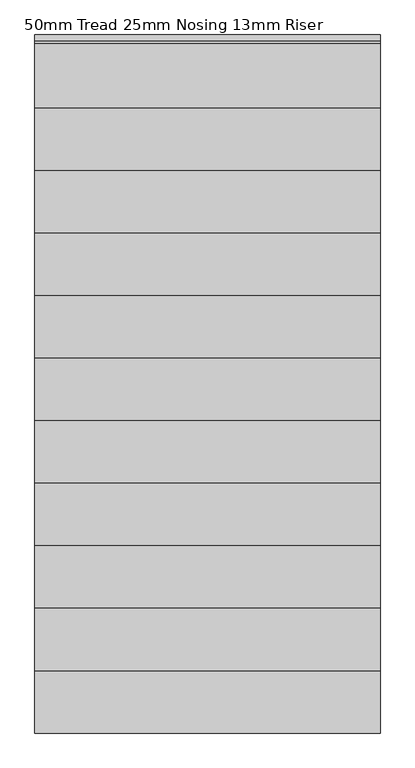
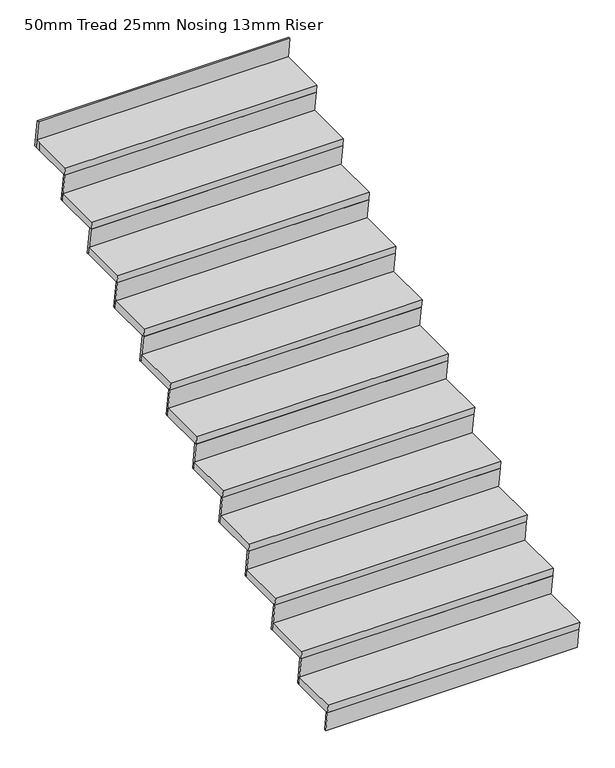
"""IFC4 building model written with IfcOpenShell, lengths in millimetres: stair flight geometry, 50mm Tread 25mm Nosing 13mm Riser."""

from ifc_helpers import new_model, si_unit, origin, place, context, project, spatial, faceted_brep, source, transform, mapped, element, save


def stair_flight_50mm_tread_25mm_nosing_13mm_riser_b2627bcb(model_context):
    return source(origin(), model_context, "Body", "Brep", [
        faceted_brep([(-499.4393676, 4584.7509075, 6676.4705882), (-499.4393676, 4591.8342409, 6626.4705882), (-2019.4393676, 4591.8342409, 6626.4705882), (-2019.4393676, 4584.7509075, 6676.4705882), (-2019.4393676, 4284.7509075, 6676.4705882), (-499.4393676, 4284.7509075, 6676.4705882), (-499.4393676, 4291.8342409, 6626.4705882), (-2019.4393676, 4291.8342409, 6626.4705882)], [[[0, 1, 2, 3]], [[3, 4, 5, 0]], [[2, 1, 6, 7]], [[4, 3, 2, 7]], [[0, 5, 6, 1]], [[5, 4, 7, 6]]]),
        faceted_brep([(-499.4393676, 4291.8342409, 6626.4705882), (-499.4393676, 4309.7509075, 6500.0), (-499.4393676, 4322.3757185, 6500.0), (-499.4393676, 4304.4590518, 6626.4705882), (-2019.4393676, 4291.8342409, 6626.4705882), (-2019.4393676, 4304.4590518, 6626.4705882), (-2019.4393676, 4322.3757185, 6500.0), (-2019.4393676, 4309.7509075, 6500.0)], [[[0, 1, 2, 3]], [[4, 5, 6, 7]], [[1, 0, 4, 7]], [[2, 1, 7, 6]], [[3, 2, 6, 5]], [[0, 3, 5, 4]]]),
        faceted_brep([(-499.4393676, 4566.8342409, 6802.9411765), (-499.4393676, 4591.8342409, 6626.4705882), (-499.4393676, 4604.4590518, 6626.4705882), (-499.4393676, 4579.4590518, 6802.9411765), (-2019.4393676, 4566.8342409, 6802.9411765), (-2019.4393676, 4579.4590518, 6802.9411765), (-2019.4393676, 4604.4590518, 6626.4705882), (-2019.4393676, 4591.8342409, 6626.4705882)], [[[0, 1, 2, 3]], [[4, 5, 6, 7]], [[1, 0, 4, 7]], [[2, 1, 7, 6]], [[3, 2, 6, 5]], [[0, 3, 5, 4]]]),
        faceted_brep([(-2019.4393676, 4859.7509075, 6852.9411765), (-2019.4393676, 4559.7509075, 6852.9411765), (-499.4393676, 4559.7509075, 6852.9411765), (-499.4393676, 4859.7509075, 6852.9411765), (-2019.4393676, 4866.8342409, 6802.9411765), (-499.4393676, 4866.8342409, 6802.9411765), (-499.4393676, 4566.8342409, 6802.9411765), (-2019.4393676, 4566.8342409, 6802.9411765)], [[[0, 1, 2, 3]], [[4, 5, 6, 7]], [[1, 0, 4, 7]], [[3, 2, 6, 5]], [[3, 5, 4, 0]], [[2, 1, 7, 6]]]),
        faceted_brep([(-499.4393676, 4841.8342409, 6979.4117647), (-499.4393676, 4866.8342409, 6802.9411765), (-499.4393676, 4879.4590518, 6802.9411765), (-499.4393676, 4854.4590518, 6979.4117647), (-2019.4393676, 4841.8342409, 6979.4117647), (-2019.4393676, 4854.4590518, 6979.4117647), (-2019.4393676, 4879.4590518, 6802.9411765), (-2019.4393676, 4866.8342409, 6802.9411765)], [[[0, 1, 2, 3]], [[4, 5, 6, 7]], [[1, 0, 4, 7]], [[2, 1, 7, 6]], [[3, 2, 6, 5]], [[0, 3, 5, 4]]]),
        faceted_brep([(-2019.4393676, 5134.7509075, 7029.4117647), (-2019.4393676, 4834.7509075, 7029.4117647), (-499.4393676, 4834.7509075, 7029.4117647), (-499.4393676, 5134.7509075, 7029.4117647), (-2019.4393676, 5141.8342409, 6979.4117647), (-499.4393676, 5141.8342409, 6979.4117647), (-499.4393676, 4841.8342409, 6979.4117647), (-2019.4393676, 4841.8342409, 6979.4117647)], [[[0, 1, 2, 3]], [[4, 5, 6, 7]], [[1, 0, 4, 7]], [[3, 2, 6, 5]], [[3, 5, 4, 0]], [[2, 1, 7, 6]]]),
        faceted_brep([(-499.4393676, 5116.8342409, 7155.8823529), (-499.4393676, 5141.8342409, 6979.4117647), (-499.4393676, 5154.4590518, 6979.4117647), (-499.4393676, 5129.4590518, 7155.8823529), (-2019.4393676, 5116.8342409, 7155.8823529), (-2019.4393676, 5129.4590518, 7155.8823529), (-2019.4393676, 5154.4590518, 6979.4117647), (-2019.4393676, 5141.8342409, 6979.4117647)], [[[0, 1, 2, 3]], [[4, 5, 6, 7]], [[1, 0, 4, 7]], [[2, 1, 7, 6]], [[3, 2, 6, 5]], [[0, 3, 5, 4]]]),
        faceted_brep([(-2019.4393676, 5409.7509075, 7205.8823529), (-2019.4393676, 5109.7509075, 7205.8823529), (-499.4393676, 5109.7509075, 7205.8823529), (-499.4393676, 5409.7509075, 7205.8823529), (-2019.4393676, 5416.8342409, 7155.8823529), (-499.4393676, 5416.8342409, 7155.8823529), (-499.4393676, 5116.8342409, 7155.8823529), (-2019.4393676, 5116.8342409, 7155.8823529)], [[[0, 1, 2, 3]], [[4, 5, 6, 7]], [[1, 0, 4, 7]], [[3, 2, 6, 5]], [[3, 5, 4, 0]], [[2, 1, 7, 6]]]),
        faceted_brep([(-499.4393676, 5391.8342409, 7332.3529412), (-499.4393676, 5416.8342409, 7155.8823529), (-499.4393676, 5429.4590518, 7155.8823529), (-499.4393676, 5404.4590518, 7332.3529412), (-2019.4393676, 5391.8342409, 7332.3529412), (-2019.4393676, 5404.4590518, 7332.3529412), (-2019.4393676, 5429.4590518, 7155.8823529), (-2019.4393676, 5416.8342409, 7155.8823529)], [[[0, 1, 2, 3]], [[4, 5, 6, 7]], [[1, 0, 4, 7]], [[2, 1, 7, 6]], [[3, 2, 6, 5]], [[0, 3, 5, 4]]]),
        faceted_brep([(-2019.4393676, 5684.7509075, 7382.3529412), (-2019.4393676, 5384.7509075, 7382.3529412), (-499.4393676, 5384.7509075, 7382.3529412), (-499.4393676, 5684.7509075, 7382.3529412), (-2019.4393676, 5691.8342409, 7332.3529412), (-499.4393676, 5691.8342409, 7332.3529412), (-499.4393676, 5391.8342409, 7332.3529412), (-2019.4393676, 5391.8342409, 7332.3529412)], [[[0, 1, 2, 3]], [[4, 5, 6, 7]], [[1, 0, 4, 7]], [[3, 2, 6, 5]], [[3, 5, 4, 0]], [[2, 1, 7, 6]]]),
        faceted_brep([(-499.4393676, 5666.8342409, 7508.8235294), (-499.4393676, 5691.8342409, 7332.3529412), (-499.4393676, 5704.4590518, 7332.3529412), (-499.4393676, 5679.4590518, 7508.8235294), (-2019.4393676, 5666.8342409, 7508.8235294), (-2019.4393676, 5679.4590518, 7508.8235294), (-2019.4393676, 5704.4590518, 7332.3529412), (-2019.4393676, 5691.8342409, 7332.3529412)], [[[0, 1, 2, 3]], [[4, 5, 6, 7]], [[1, 0, 4, 7]], [[2, 1, 7, 6]], [[3, 2, 6, 5]], [[0, 3, 5, 4]]]),
        faceted_brep([(-2019.4393676, 5959.7509075, 7558.8235294), (-2019.4393676, 5659.7509075, 7558.8235294), (-499.4393676, 5659.7509075, 7558.8235294), (-499.4393676, 5959.7509075, 7558.8235294), (-2019.4393676, 5966.8342409, 7508.8235294), (-499.4393676, 5966.8342409, 7508.8235294), (-499.4393676, 5666.8342409, 7508.8235294), (-2019.4393676, 5666.8342409, 7508.8235294)], [[[0, 1, 2, 3]], [[4, 5, 6, 7]], [[1, 0, 4, 7]], [[3, 2, 6, 5]], [[3, 5, 4, 0]], [[2, 1, 7, 6]]]),
        faceted_brep([(-499.4393676, 5941.8342409, 7685.2941176), (-499.4393676, 5966.8342409, 7508.8235294), (-499.4393676, 5979.4590518, 7508.8235294), (-499.4393676, 5954.4590518, 7685.2941176), (-2019.4393676, 5941.8342409, 7685.2941176), (-2019.4393676, 5954.4590518, 7685.2941176), (-2019.4393676, 5979.4590518, 7508.8235294), (-2019.4393676, 5966.8342409, 7508.8235294)], [[[0, 1, 2, 3]], [[4, 5, 6, 7]], [[1, 0, 4, 7]], [[2, 1, 7, 6]], [[3, 2, 6, 5]], [[0, 3, 5, 4]]]),
        faceted_brep([(-2019.4393676, 6234.7509075, 7735.2941176), (-2019.4393676, 5934.7509075, 7735.2941176), (-499.4393676, 5934.7509075, 7735.2941176), (-499.4393676, 6234.7509075, 7735.2941176), (-2019.4393676, 6241.8342409, 7685.2941176), (-499.4393676, 6241.8342409, 7685.2941176), (-499.4393676, 5941.8342409, 7685.2941176), (-2019.4393676, 5941.8342409, 7685.2941176)], [[[0, 1, 2, 3]], [[4, 5, 6, 7]], [[1, 0, 4, 7]], [[3, 2, 6, 5]], [[3, 5, 4, 0]], [[2, 1, 7, 6]]]),
        faceted_brep([(-499.4393676, 6216.8342409, 7861.7647059), (-499.4393676, 6241.8342409, 7685.2941176), (-499.4393676, 6254.4590518, 7685.2941176), (-499.4393676, 6229.4590518, 7861.7647059), (-2019.4393676, 6216.8342409, 7861.7647059), (-2019.4393676, 6229.4590518, 7861.7647059), (-2019.4393676, 6254.4590518, 7685.2941176), (-2019.4393676, 6241.8342409, 7685.2941176)], [[[0, 1, 2, 3]], [[4, 5, 6, 7]], [[1, 0, 4, 7]], [[2, 1, 7, 6]], [[3, 2, 6, 5]], [[0, 3, 5, 4]]]),
        faceted_brep([(-2019.4393676, 6509.7509075, 7911.7647059), (-2019.4393676, 6209.7509075, 7911.7647059), (-499.4393676, 6209.7509075, 7911.7647059), (-499.4393676, 6509.7509075, 7911.7647059), (-2019.4393676, 6516.8342409, 7861.7647059), (-499.4393676, 6516.8342409, 7861.7647059), (-499.4393676, 6216.8342409, 7861.7647059), (-2019.4393676, 6216.8342409, 7861.7647059)], [[[0, 1, 2, 3]], [[4, 5, 6, 7]], [[1, 0, 4, 7]], [[3, 2, 6, 5]], [[3, 5, 4, 0]], [[2, 1, 7, 6]]]),
        faceted_brep([(-499.4393676, 6491.8342409, 8038.2352941), (-499.4393676, 6516.8342409, 7861.7647059), (-499.4393676, 6529.4590518, 7861.7647059), (-499.4393676, 6504.4590518, 8038.2352941), (-2019.4393676, 6491.8342409, 8038.2352941), (-2019.4393676, 6504.4590518, 8038.2352941), (-2019.4393676, 6529.4590518, 7861.7647059), (-2019.4393676, 6516.8342409, 7861.7647059)], [[[0, 1, 2, 3]], [[4, 5, 6, 7]], [[1, 0, 4, 7]], [[2, 1, 7, 6]], [[3, 2, 6, 5]], [[0, 3, 5, 4]]]),
        faceted_brep([(-2019.4393676, 6784.7509075, 8088.2352941), (-2019.4393676, 6484.7509075, 8088.2352941), (-499.4393676, 6484.7509075, 8088.2352941), (-499.4393676, 6784.7509075, 8088.2352941), (-2019.4393676, 6791.8342409, 8038.2352941), (-499.4393676, 6791.8342409, 8038.2352941), (-499.4393676, 6491.8342409, 8038.2352941), (-2019.4393676, 6491.8342409, 8038.2352941)], [[[0, 1, 2, 3]], [[4, 5, 6, 7]], [[1, 0, 4, 7]], [[3, 2, 6, 5]], [[3, 5, 4, 0]], [[2, 1, 7, 6]]]),
        faceted_brep([(-499.4393676, 6766.8342409, 8214.7058824), (-499.4393676, 6791.8342409, 8038.2352941), (-499.4393676, 6804.4590518, 8038.2352941), (-499.4393676, 6779.4590518, 8214.7058824), (-2019.4393676, 6766.8342409, 8214.7058824), (-2019.4393676, 6779.4590518, 8214.7058824), (-2019.4393676, 6804.4590518, 8038.2352941), (-2019.4393676, 6791.8342409, 8038.2352941)], [[[0, 1, 2, 3]], [[4, 5, 6, 7]], [[1, 0, 4, 7]], [[2, 1, 7, 6]], [[3, 2, 6, 5]], [[0, 3, 5, 4]]]),
        faceted_brep([(-2019.4393676, 7059.7509075, 8264.7058824), (-2019.4393676, 6759.7509075, 8264.7058824), (-499.4393676, 6759.7509075, 8264.7058824), (-499.4393676, 7059.7509075, 8264.7058824), (-2019.4393676, 7066.8342409, 8214.7058824), (-499.4393676, 7066.8342409, 8214.7058824), (-499.4393676, 6766.8342409, 8214.7058824), (-2019.4393676, 6766.8342409, 8214.7058824)], [[[0, 1, 2, 3]], [[4, 5, 6, 7]], [[1, 0, 4, 7]], [[3, 2, 6, 5]], [[3, 5, 4, 0]], [[2, 1, 7, 6]]]),
        faceted_brep([(-499.4393676, 7316.8342409, 8567.6470588), (-499.4393676, 7341.8342409, 8391.1764706), (-499.4393676, 7354.4590518, 8391.1764706), (-499.4393676, 7329.4590518, 8567.6470588), (-2019.4393676, 7316.8342409, 8567.6470588), (-2019.4393676, 7329.4590518, 8567.6470588), (-2019.4393676, 7354.4590518, 8391.1764706), (-2019.4393676, 7341.8342409, 8391.1764706)], [[[0, 1, 2, 3]], [[4, 5, 6, 7]], [[1, 0, 4, 7]], [[2, 1, 7, 6]], [[3, 2, 6, 5]], [[0, 3, 5, 4]]]),
        faceted_brep([(-499.4393676, 7041.8342409, 8391.1764706), (-499.4393676, 7066.8342409, 8214.7058824), (-499.4393676, 7079.4590518, 8214.7058824), (-499.4393676, 7054.4590518, 8391.1764706), (-2019.4393676, 7041.8342409, 8391.1764706), (-2019.4393676, 7054.4590518, 8391.1764706), (-2019.4393676, 7079.4590518, 8214.7058824), (-2019.4393676, 7066.8342409, 8214.7058824)], [[[0, 1, 2, 3]], [[4, 5, 6, 7]], [[1, 0, 4, 7]], [[2, 1, 7, 6]], [[3, 2, 6, 5]], [[0, 3, 5, 4]]]),
        faceted_brep([(-2019.4393676, 7334.7509075, 8441.1764706), (-2019.4393676, 7309.7509075, 8441.1764706), (-2019.4393676, 7034.7509075, 8441.1764706), (-499.4393676, 7034.7509075, 8441.1764706), (-499.4393676, 7334.7509075, 8441.1764706), (-2019.4393676, 7341.8342409, 8391.1764706), (-499.4393676, 7341.8342409, 8391.1764706), (-499.4393676, 7041.8342409, 8391.1764706), (-2019.4393676, 7041.8342409, 8391.1764706), (-2019.4393676, 7309.7509075, 8391.1764706)], [[[0, 1, 2, 3, 4]], [[5, 6, 7, 8, 9]], [[1, 0, 5, 9]], [[2, 1, 9, 8]], [[4, 3, 7, 6]], [[4, 6, 5, 0]], [[3, 2, 8, 7]]]),
    ])


if __name__ == "__main__":
    model = new_model("IFC4")
    model_context = context("Model", 3, world=origin())
    ifc_project = project(units=[si_unit("LENGTHUNIT", "METRE", prefix="MILLI")], contexts=[model_context])
    site = spatial("IfcSite", under=ifc_project)
    building = spatial("IfcBuilding", under=site)
    placement = place(None, origin())
    stair_flight_50mm_tread_25mm_nosing_13mm_riser_shape = stair_flight_50mm_tread_25mm_nosing_13mm_riser_b2627bcb(model_context)
    element("IfcStairFlight", 1, ObjectType="50mm Tread 25mm Nosing 13mm Riser", at=placement, inside=building, context=model_context, shape_type="MappedRepresentation", body=[
        mapped(stair_flight_50mm_tread_25mm_nosing_13mm_riser_shape, transform((0.0, 0.0, 0.0), x_axis=(1.0, 0.0, 0.0), y_axis=(0.0, 1.0, 0.0), z_axis=(0.0, 0.0, 1.0))),
    ])
    save(model, "model.ifc")
